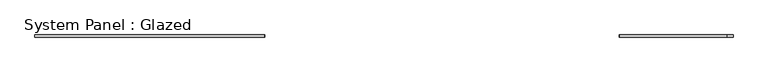
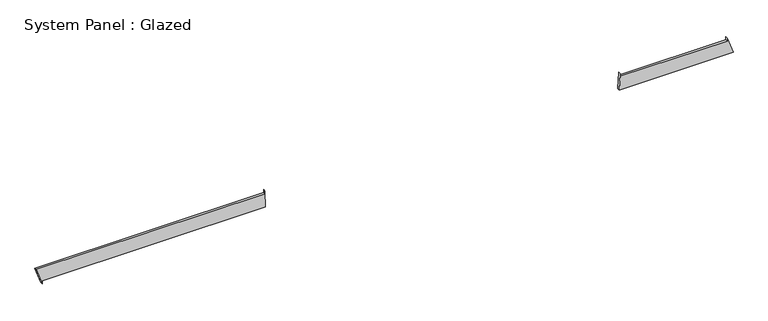
"""IFC4 building model written with IfcOpenShell, lengths in millimetres: plate geometry, System Panel : Glazed."""

from ifc_helpers import new_model, si_unit, frame, origin, place, context, project, spatial, polyline, outline, extrude, source, transform, mapped, element, save


def system_panel_glazed_a1e72640(model_context):
    return source(origin(), model_context, "Body", "SweptSolid", [
        extrude(outline(polyline([(0.0, -3958.5507161), (35.3553391, -3958.5507161), (35.3553391, -1377.5436269), (234.6939562, -1382.7201119), (199.3386172, -1382.7194789), (199.2912695, -4027.4801939), (0.0, -3958.5507161)])), frame((0.0, -49.5, 0.0), z_axis=(0.0, 1.0, 0.0), x_axis=(0.0, 0.0, 1.0)), (0.0, 0.0, 1.0), 25.0),
        extrude(outline(polyline([(35.3553391, 2711.6809934), (35.3553391, 4027.4801939), (234.7895843, 3958.8960097), (199.4342452, 3958.8966426), (199.4121015, 2721.9901772), (234.7674406, 2721.9895442), (35.3553391, 2711.6809934)])), frame((0.0, -49.5, 0.0), z_axis=(0.0, 1.0, 0.0), x_axis=(0.0, 0.0, 1.0)), (0.0, 0.0, 1.0), 25.0),
    ])


if __name__ == "__main__":
    model = new_model("IFC4")
    model_context = context("Model", 3, world=origin())
    ifc_project = project(units=[si_unit("LENGTHUNIT", "METRE", prefix="MILLI")], contexts=[model_context])
    site = spatial("IfcSite", under=ifc_project)
    building = spatial("IfcBuilding", under=site)
    placement = place(None, origin())
    system_panel_glazed_shape = system_panel_glazed_a1e72640(model_context)
    element("IfcPlate", 1, ObjectType="System Panel : Glazed", at=placement, inside=building, context=model_context, shape_type="MappedRepresentation", body=[
        mapped(system_panel_glazed_shape, transform((0.0, 0.0, 0.0), x_axis=(1.0, 0.0, 0.0), y_axis=(0.0, 1.0, 0.0), z_axis=(0.0, 0.0, 1.0))),
    ])
    save(model, "model.ifc")

# Revit data of these elements
# Element 1 (IfcPlate, "System Panel : Glazed")
#   Materials on its faces: "Glass"
# Materials
#   "Glass": class "Glass", colour RGB 218 227 224, transparency 0.85, Description = "Soda Lime Glass", Cost = 0
